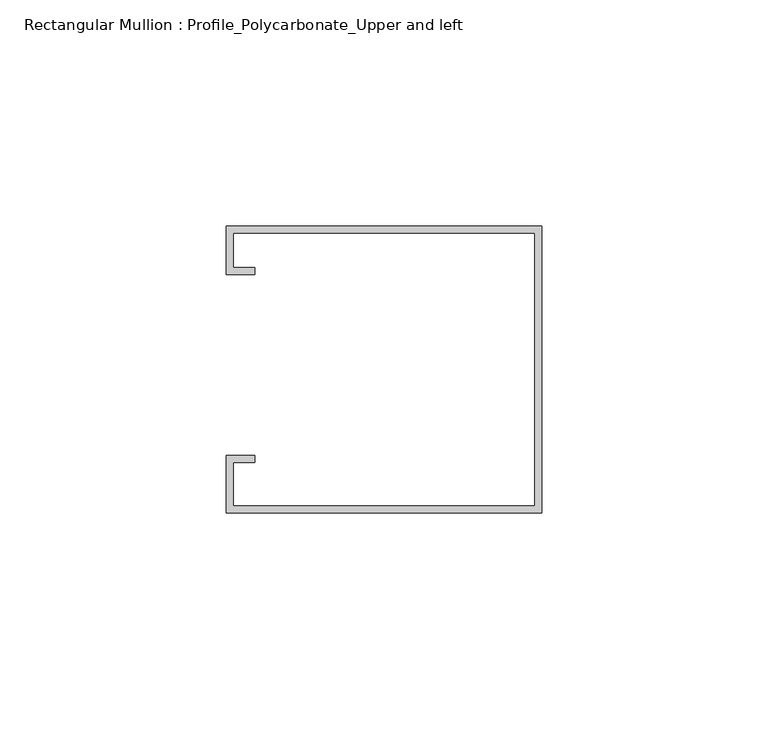
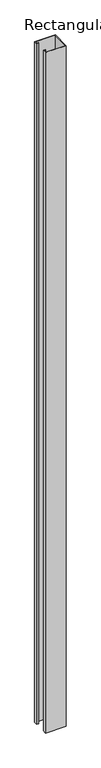
"""IFC4 building model written with IfcOpenShell, lengths in millimetres: member geometry, Rectangular Mullion : Profile_Polycarbonate_Upper and left."""

from ifc_helpers import new_model, si_unit, frame, origin, place, context, project, spatial, polyline, outline, extrude, source, transform, mapped, element, save


def rectangular_mullion_profile_polycarbonate_upper_and_left_dbc7a052(model_context):
    return source(origin(), model_context, "Body", "SweptSolid", [
        extrude(outline(polyline([(0.0, -32.7), (-69.85, -32.7), (-69.85, -20.0), (-63.5, -20.0), (-63.5, -21.5875), (-68.2625, -21.5875), (-68.2625, -31.1125), (-1.5875, -31.1125), (-1.5875, 29.2125), (-68.2625, 29.2125), (-68.2625, 21.5875), (-63.5, 21.5875), (-63.5, 20.0), (-69.85, 20.0), (-69.85, 30.8), (0.0, 30.8), (0.0, -32.7)])), frame((0.0, 0.0, -2438.4), z_axis=(0.0, 0.0, 1.0), x_axis=(1.0, 0.0, 0.0)), (0.0, 0.0, 1.0), 2438.4),
    ])


if __name__ == "__main__":
    model = new_model("IFC4")
    model_context = context("Model", 3, world=origin())
    ifc_project = project(units=[si_unit("LENGTHUNIT", "METRE", prefix="MILLI")], contexts=[model_context])
    site = spatial("IfcSite", under=ifc_project)
    building = spatial("IfcBuilding", under=site)
    placement = place(None, origin())
    rectangular_mullion_profile_polycarbonate_upper_and_left_shape = rectangular_mullion_profile_polycarbonate_upper_and_left_dbc7a052(model_context)
    element("IfcMember", 1, ObjectType="Rectangular Mullion : Profile_Polycarbonate_Upper and left", at=placement, inside=building, context=model_context, shape_type="MappedRepresentation", body=[
        mapped(rectangular_mullion_profile_polycarbonate_upper_and_left_shape, transform((0.0, 0.0, 0.0), x_axis=(1.0, 0.0, 0.0), y_axis=(0.0, 1.0, 0.0), z_axis=(0.0, 0.0, 1.0))),
    ])
    save(model, "model.ifc")

# Revit data of these elements
# Type "Rectangular Mullion : Profile_Polycarbonate_Upper and left"
#   built-in parameter 1007322 = 0.208333 (stored number, unit not read)
#   built-in parameter 1007321 = 0.00520833 (stored number, unit not read)
#   built-in parameter 1007320 = 0 (stored number, unit not read)
# Element 1 (IfcMember, "Rectangular Mullion : Profile_Polycarbonate_Upper and left")
#   Materials on its faces: "Aluminum"
# Materials
#   "Aluminum": class "Metal", colour RGB 244 244 244, transparency 0, Description = "Aluminum 6061", Cost = 0
